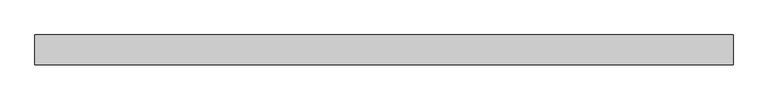
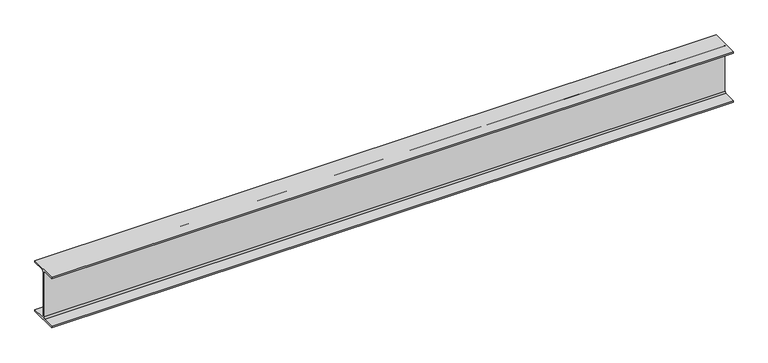
"""IFC4 building model written with IfcOpenShell, lengths in millimetres: beam geometry, Old_Steel Beam_H-KSD3502 : H_SB_ASB_H-250×125x6x9."""

import ifcopenshell
import ifcopenshell.guid

model = None  # the IFC model being written
_history = None  # IfcOwnerHistory: only IFC2X3 demands one
_inside = {}  # id of a spatial element -> (the spatial element, [elements in it])
_under = {}  # id of a project, library or spatial element -> (it, [spatial elements below it])
_declared = {}  # id of a project -> (the project, [libraries it declares])
_typed = {}  # id of a type object -> (the type object, [elements of that type])
_made_of = {}  # id of a material, layer set ... -> (it, [elements and type objects made of it])


def new_model(schema):
    """Start an empty IFC model of exactly this schema.

    Asked for "IFC4X3", IfcOpenShell would pick the latest addendum, in which some entities
    have other attributes; the version numbers below select the first issue.
    IFC2X3 requires an IfcOwnerHistory on every rooted entity: one is made here for all.
    """
    global model, _history
    if schema == "IFC4X3":
        model = ifcopenshell.file(schema_version=(4, 3, 0, 0))
    else:
        model = ifcopenshell.file(schema=schema)
    _inside.clear()
    _under.clear()
    _declared.clear()
    _typed.clear()
    _made_of.clear()
    _history = None
    if model.schema == "IFC2X3":
        org = make("IfcOrganization", Name="unknown")
        user = make(
            "IfcPersonAndOrganization",
            ThePerson=make("IfcPerson", FamilyName="unknown"),
            TheOrganization=org,
        )
        app = make(
            "IfcApplication",
            ApplicationDeveloper=org,
            Version="unknown",
            ApplicationFullName="unknown",
            ApplicationIdentifier="unknown",
        )
        _history = make(
            "IfcOwnerHistory",
            OwningUser=user,
            OwningApplication=app,
            ChangeAction="ADDED",
            CreationDate=0,
        )
    return model


def make(cls, **values):
    """One entity of the class cls with the attributes given. An attribute that is None is left unset."""
    return model.create_entity(
        cls, **{name: value for name, value in values.items() if value is not None}
    )


def rooted(cls, **values):
    """An entity with a GlobalId (a new one), such as an element, a storey or a relation."""
    return make(cls, GlobalId=ifcopenshell.guid.new(), OwnerHistory=_history, **values)


def si_unit(unit_type, name, prefix=None):
    """IfcSIUnit, for example si_unit("LENGTHUNIT", "METRE", prefix="MILLI")."""
    return make("IfcSIUnit", UnitType=unit_type, Prefix=prefix, Name=name)


def assignment(units):
    """IfcUnitAssignment: the units of a project."""
    return None if units is None else make("IfcUnitAssignment", Units=units)


def point(xyz):
    """IfcCartesianPoint."""
    return None if xyz is None else make("IfcCartesianPoint", Coordinates=xyz)


def direction(xyz):
    """IfcDirection."""
    return None if xyz is None else make("IfcDirection", DirectionRatios=xyz)


def frame(location, z_axis=None, x_axis=None):
    """IfcAxis2Placement3D, a coordinate frame: its origin and axes. An axis left out is left unset."""
    return make(
        "IfcAxis2Placement3D",
        Location=point(location),
        Axis=direction(z_axis),
        RefDirection=direction(x_axis),
    )


def frame_2d(location, x_axis=None):
    """IfcAxis2Placement2D, a coordinate frame in the plane: its origin and x axis."""
    return make(
        "IfcAxis2Placement2D", Location=point(location), RefDirection=direction(x_axis)
    )


def origin():
    """The frame at (0, 0, 0) with its axes left unset."""
    return frame((0.0, 0.0, 0.0))


def place(relative_to, where):
    """IfcLocalPlacement: puts the frame where relative to a parent placement (None: the world)."""
    return make(
        "IfcLocalPlacement", PlacementRelTo=relative_to, RelativePlacement=where
    )


def context(
    kind, dimensions, precision=None, world=None, true_north=None, identifier=None
):
    """IfcGeometricRepresentationContext, for example the 3D "Model" context."""
    return make(
        "IfcGeometricRepresentationContext",
        ContextIdentifier=identifier,
        ContextType=kind,
        CoordinateSpaceDimension=dimensions,
        Precision=precision,
        WorldCoordinateSystem=world,
        TrueNorth=true_north,
    )


def project(units=None, contexts=None):
    """IfcProject with its units and contexts."""
    return rooted(
        "IfcProject",
        Name="project",
        RepresentationContexts=contexts,
        UnitsInContext=assignment(units),
    )


def spatial(cls, under=None, at=None, **own):
    """A site, building, storey or space (cls), placed at a placement, below another one or the project."""
    s = rooted(cls, ObjectPlacement=at, **own)
    if under is not None:
        _under.setdefault(under.id(), (under, []))[1].append(s)
    return s


def polyline(points):
    """IfcPolyline through the points."""
    return make("IfcPolyline", Points=[point(p) for p in points])


def circle_curve(where, radius):
    """IfcCircle in the frame where."""
    return make("IfcCircle", Position=where, Radius=radius)


def trimmed(basis, trim1, trim2, sense, master):
    """IfcTrimmedCurve: the piece of a basis curve between two trims."""
    return make(
        "IfcTrimmedCurve",
        BasisCurve=basis,
        Trim1=trim1,
        Trim2=trim2,
        SenseAgreement=sense,
        MasterRepresentation=master,
    )


def segment(curve, same_sense, transition):
    """IfcCompositeCurveSegment."""
    return make(
        "IfcCompositeCurveSegment",
        Transition=transition,
        SameSense=same_sense,
        ParentCurve=curve,
    )


def composite_curve(segments, self_intersect=None):
    """IfcCompositeCurve: segments joined end to end."""
    return make("IfcCompositeCurve", Segments=segments, SelfIntersect=self_intersect)


def outline(outer, holes=None, kind="AREA"):
    """IfcArbitraryClosedProfileDef: a profile drawn as a closed curve; with holes, ...WithVoids."""
    if holes is None:
        return make("IfcArbitraryClosedProfileDef", ProfileType=kind, OuterCurve=outer)
    return make(
        "IfcArbitraryProfileDefWithVoids",
        ProfileType=kind,
        OuterCurve=outer,
        InnerCurves=holes,
    )


def extrude(swept, where, along, depth):
    """IfcExtrudedAreaSolid: the profile swept, set in the frame where, extruded along a direction by depth."""
    return make(
        "IfcExtrudedAreaSolid",
        SweptArea=swept,
        Position=where,
        ExtrudedDirection=direction(along),
        Depth=depth,
    )


def shape(context_of_items, identifier, shape_type, items):
    """IfcShapeRepresentation: the items that make up one representation, for example the "Body"."""
    return make(
        "IfcShapeRepresentation",
        ContextOfItems=context_of_items,
        RepresentationIdentifier=identifier,
        RepresentationType=shape_type,
        Items=items,
    )


def source(mapping_origin, context_of_items, identifier, shape_type, items):
    """IfcRepresentationMap: a shape defined once, which mapped items show again and again."""
    return make(
        "IfcRepresentationMap",
        MappingOrigin=mapping_origin,
        MappedRepresentation=shape(context_of_items, identifier, shape_type, items),
    )


def transform(
    local_origin,
    x_axis=None,
    y_axis=None,
    z_axis=None,
    scale=None,
    scale2=None,
    scale3=None,
    uniform=True,
):
    """IfcCartesianTransformationOperator3D, or its non-uniform kind. x_axis, y_axis, z_axis: its Axis1, 2, 3."""
    if uniform:
        return make(
            "IfcCartesianTransformationOperator3D",
            Axis1=direction(x_axis),
            Axis2=direction(y_axis),
            LocalOrigin=point(local_origin),
            Scale=scale,
            Axis3=direction(z_axis),
        )
    return make(
        "IfcCartesianTransformationOperator3DnonUniform",
        Axis1=direction(x_axis),
        Axis2=direction(y_axis),
        LocalOrigin=point(local_origin),
        Scale=scale,
        Axis3=direction(z_axis),
        Scale2=scale2,
        Scale3=scale3,
    )


def mapped(mapping_source, mapping_target):
    """IfcMappedItem: shows the shape of a source again, moved by a transform."""
    return make(
        "IfcMappedItem", MappingSource=mapping_source, MappingTarget=mapping_target
    )


def made_of(thing, what):
    """Note that an element or type object is made of a material, layer set ...; save() writes the relation."""
    if what is not None:
        _made_of.setdefault(what.id(), (what, []))[1].append(thing)
    return thing


def element(
    cls,
    number,
    at=None,
    inside=None,
    cuts=None,
    type_object=None,
    material=None,
    context=None,
    identifier="Body",
    shape_type=None,
    held_by="IfcProductDefinitionShape",
    body=None,
    shapes=None,
    **own,
):
    """One element of the class cls, such as IfcWall. Its Tag is "e" and its number.

    at: its placement. inside: the storey or other place that contains it. cuts: it is an
    opening in that element (IfcRelVoidsElement). A single representation is given by context,
    identifier, shape_type and body (its items); several are given by shapes. held_by: the class
    of the entity that holds the representations. save() writes the other relations.
    """
    e = rooted(cls, Tag="e%d" % number, ObjectPlacement=at, **own)
    if body is not None:
        shapes = [shape(context, identifier, shape_type, body)]
    if shapes is not None:
        e.Representation = make(held_by, Representations=shapes)
    if inside is not None:
        _inside.setdefault(inside.id(), (inside, []))[1].append(e)
    if cuts is not None:
        rooted(
            "IfcRelVoidsElement", RelatingBuildingElement=cuts, RelatedOpeningElement=e
        )
    if type_object is not None:
        _typed.setdefault(type_object.id(), (type_object, []))[1].append(e)
    return made_of(e, material)


def aggregate(whole, parts):
    """IfcRelAggregates: a whole, such as a stair, and the parts it consists of."""
    return rooted("IfcRelAggregates", RelatingObject=whole, RelatedObjects=parts)


def save(model, path):
    """Write the relations noted so far, then the file.

    IfcRelAggregates (storeys below a building ...), IfcRelContainedInSpatialStructure (elements
    in a storey), IfcRelDefinesByType, IfcRelAssociatesMaterial and IfcRelDeclares: one each for
    every whole, place, type object, material and project.
    """
    for whole, parts in _under.values():
        aggregate(whole, parts)
    for where, things in _inside.values():
        rooted(
            "IfcRelContainedInSpatialStructure",
            RelatedElements=things,
            RelatingStructure=where,
        )
    for kind, things in _typed.values():
        rooted("IfcRelDefinesByType", RelatedObjects=things, RelatingType=kind)
    for what, things in _made_of.values():
        rooted("IfcRelAssociatesMaterial", RelatedObjects=things, RelatingMaterial=what)
    for by, libraries in _declared.values():
        rooted("IfcRelDeclares", RelatingContext=by, RelatedDefinitions=libraries)
    model.write(path)


def beam_5c55ab62(model_context):
    return source(origin(), model_context, "Body", "SweptSolid", [
        extrude(outline(composite_curve([segment(polyline([(82.5, -141.5), (82.5, -151.7), (-82.5, -151.7), (-82.5, -141.5), (-11.9, -141.5)]), True, "CONTINUOUS"), segment(trimmed(circle_curve(frame_2d((-11.9, -132.6)), 8.9), [point((-11.9, -141.5))], [point((-3.0, -132.6))], True, "CARTESIAN"), True, "CONTINUOUS"), segment(polyline([(-3.0, -132.6), (-3.0, 132.6)]), True, "CONTINUOUS"), segment(trimmed(circle_curve(frame_2d((-11.9, 132.6)), 8.9), [point((-3.0, 132.6))], [point((-11.9, 141.5))], True, "CARTESIAN"), True, "CONTINUOUS"), segment(polyline([(-11.9, 141.5), (-82.5, 141.5), (-82.5, 151.7), (82.5, 151.7), (82.5, 141.5), (11.9, 141.5)]), True, "CONTINUOUS"), segment(trimmed(circle_curve(frame_2d((11.9, 132.6)), 8.9), [point((11.9, 141.5))], [point((3.0, 132.6))], True, "CARTESIAN"), True, "CONTINUOUS"), segment(polyline([(3.0, 132.6), (3.0, -132.6)]), True, "CONTINUOUS"), segment(trimmed(circle_curve(frame_2d((11.9, -132.6)), 8.9), [point((3.0, -132.6))], [point((11.9, -141.5))], True, "CARTESIAN"), True, "CONTINUOUS"), segment(polyline([(11.9, -141.5), (82.5, -141.5)]), True, "CONTINUOUS")], self_intersect=False)), frame((-1830.0829189, 0.0, 0.0), z_axis=(1.0, 0.0, 0.0), x_axis=(0.0, 1.0, 0.0)), (0.0, 0.0, 1.0), 3859.8829189),
    ])


if __name__ == "__main__":
    model = new_model("IFC4")
    model_context = context("Model", 3, world=origin())
    ifc_project = project(units=[si_unit("LENGTHUNIT", "METRE", prefix="MILLI")], contexts=[model_context])
    site = spatial("IfcSite", under=ifc_project)
    building = spatial("IfcBuilding", under=site)
    placement = place(None, origin())
    beam_shape = beam_5c55ab62(model_context)
    element("IfcBeam", 1, ObjectType="Old_Steel Beam_H-KSD3502 : H_SB_ASB_H-250×125x6x9", at=placement, inside=building, context=model_context, shape_type="MappedRepresentation", body=[
        mapped(beam_shape, transform((0.0, 0.0, 0.0), x_axis=(1.0, 0.0, 0.0), y_axis=(0.0, 1.0, 0.0), z_axis=(0.0, 0.0, 1.0))),
    ])
    save(model, "model.ifc")

# Revit data of these elements
# Type "Old_Steel Beam_H-KSD3502 : H_SB_ASB_H-250×125x6x9"
#   Width = 12.5 cm
#   Web Thickness = 0.6 cm
#   Web Fillet = 1.2 cm
#   Warping Constant = 42539.8 cm⁶
#   Torsional Moment of Inertia = 7.8102 cm⁴
#   Torsional Modulus = 1.0 cm³
#   Section Area = 37.66 cm²
#   Plastic Modulus weak axis = 73.1 cm³
#   Plastic Modulus strong axis = 366.0 cm³
#   Perimeter = 0.97 m²/m
#   Nominal Weight = 29.60 kgf/m
#   Moment of Inertia weak axis = 294.00 cm⁴
#   Moment of Inertia strong axis = 4050.00 cm⁴
#   Height = 25.0 cm
#   Flange Thickness = 0.9 cm
#   Elastic Modulus weak axis = 47.0 cm³
#   Elastic Modulus strong axis = 324.0 cm³
#   Centroid Vertical = 12.5 cm
#   Centroid Horizontal = 6.25 cm
#   Length [instance default] = 1.5240 m
#   Structural Material [instance default] = Steel, 45-345
#   Assembly Code = ""
# Element 1 (IfcBeam, "Old_Steel Beam_H-KSD3502 : H_SB_ASB_H-250×125x6x9")
#   Structural Material = none
# Materials
#   "Steel, 45-345": class "Metal", colour RGB 189 187 185, transparency 0, Description = "Steel 345 MPa", Cost = 0
